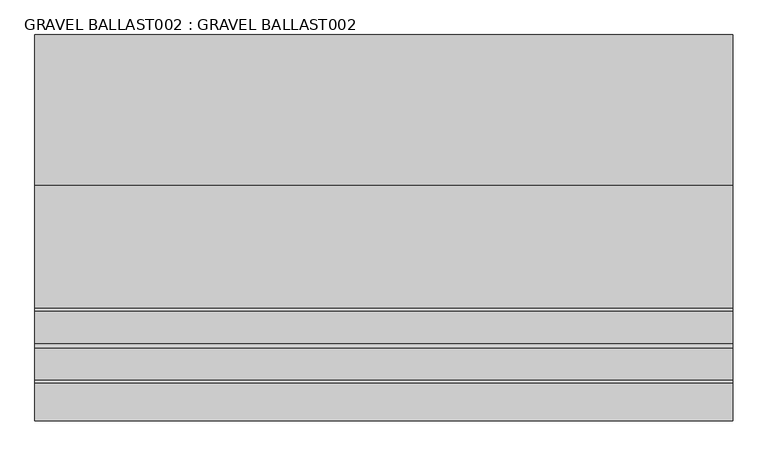
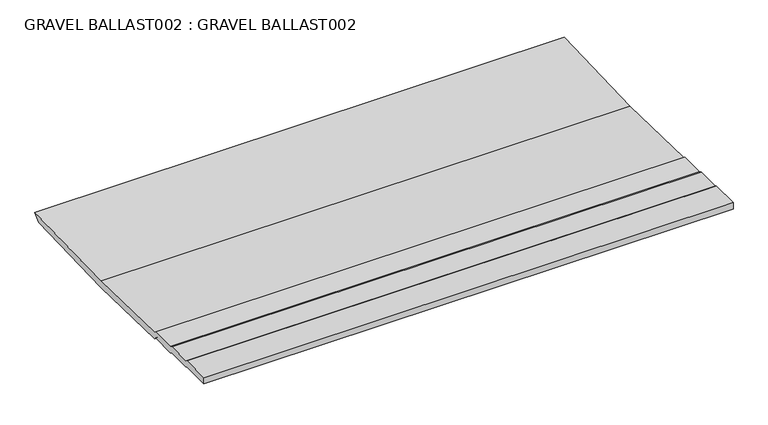
"""IFC4 building model written with IfcOpenShell, lengths in millimetres: proxy geometry, GRAVEL BALLAST002 : GRAVEL BALLAST002."""

import ifcopenshell
import ifcopenshell.guid

model = None  # the IFC model being written
_history = None  # IfcOwnerHistory: only IFC2X3 demands one
_inside = {}  # id of a spatial element -> (the spatial element, [elements in it])
_under = {}  # id of a project, library or spatial element -> (it, [spatial elements below it])
_declared = {}  # id of a project -> (the project, [libraries it declares])
_typed = {}  # id of a type object -> (the type object, [elements of that type])
_made_of = {}  # id of a material, layer set ... -> (it, [elements and type objects made of it])


def new_model(schema):
    """Start an empty IFC model of exactly this schema.

    Asked for "IFC4X3", IfcOpenShell would pick the latest addendum, in which some entities
    have other attributes; the version numbers below select the first issue.
    IFC2X3 requires an IfcOwnerHistory on every rooted entity: one is made here for all.
    """
    global model, _history
    if schema == "IFC4X3":
        model = ifcopenshell.file(schema_version=(4, 3, 0, 0))
    else:
        model = ifcopenshell.file(schema=schema)
    _inside.clear()
    _under.clear()
    _declared.clear()
    _typed.clear()
    _made_of.clear()
    _history = None
    if model.schema == "IFC2X3":
        org = make("IfcOrganization", Name="unknown")
        user = make(
            "IfcPersonAndOrganization",
            ThePerson=make("IfcPerson", FamilyName="unknown"),
            TheOrganization=org,
        )
        app = make(
            "IfcApplication",
            ApplicationDeveloper=org,
            Version="unknown",
            ApplicationFullName="unknown",
            ApplicationIdentifier="unknown",
        )
        _history = make(
            "IfcOwnerHistory",
            OwningUser=user,
            OwningApplication=app,
            ChangeAction="ADDED",
            CreationDate=0,
        )
    return model


def make(cls, **values):
    """One entity of the class cls with the attributes given. An attribute that is None is left unset."""
    return model.create_entity(
        cls, **{name: value for name, value in values.items() if value is not None}
    )


def rooted(cls, **values):
    """An entity with a GlobalId (a new one), such as an element, a storey or a relation."""
    return make(cls, GlobalId=ifcopenshell.guid.new(), OwnerHistory=_history, **values)


def si_unit(unit_type, name, prefix=None):
    """IfcSIUnit, for example si_unit("LENGTHUNIT", "METRE", prefix="MILLI")."""
    return make("IfcSIUnit", UnitType=unit_type, Prefix=prefix, Name=name)


def assignment(units):
    """IfcUnitAssignment: the units of a project."""
    return None if units is None else make("IfcUnitAssignment", Units=units)


def point(xyz):
    """IfcCartesianPoint."""
    return None if xyz is None else make("IfcCartesianPoint", Coordinates=xyz)


def direction(xyz):
    """IfcDirection."""
    return None if xyz is None else make("IfcDirection", DirectionRatios=xyz)


def frame(location, z_axis=None, x_axis=None):
    """IfcAxis2Placement3D, a coordinate frame: its origin and axes. An axis left out is left unset."""
    return make(
        "IfcAxis2Placement3D",
        Location=point(location),
        Axis=direction(z_axis),
        RefDirection=direction(x_axis),
    )


def origin():
    """The frame at (0, 0, 0) with its axes left unset."""
    return frame((0.0, 0.0, 0.0))


def place(relative_to, where):
    """IfcLocalPlacement: puts the frame where relative to a parent placement (None: the world)."""
    return make(
        "IfcLocalPlacement", PlacementRelTo=relative_to, RelativePlacement=where
    )


def context(
    kind, dimensions, precision=None, world=None, true_north=None, identifier=None
):
    """IfcGeometricRepresentationContext, for example the 3D "Model" context."""
    return make(
        "IfcGeometricRepresentationContext",
        ContextIdentifier=identifier,
        ContextType=kind,
        CoordinateSpaceDimension=dimensions,
        Precision=precision,
        WorldCoordinateSystem=world,
        TrueNorth=true_north,
    )


def project(units=None, contexts=None):
    """IfcProject with its units and contexts."""
    return rooted(
        "IfcProject",
        Name="project",
        RepresentationContexts=contexts,
        UnitsInContext=assignment(units),
    )


def spatial(cls, under=None, at=None, **own):
    """A site, building, storey or space (cls), placed at a placement, below another one or the project."""
    s = rooted(cls, ObjectPlacement=at, **own)
    if under is not None:
        _under.setdefault(under.id(), (under, []))[1].append(s)
    return s


def polyline(points):
    """IfcPolyline through the points."""
    return make("IfcPolyline", Points=[point(p) for p in points])


def outline(outer, holes=None, kind="AREA"):
    """IfcArbitraryClosedProfileDef: a profile drawn as a closed curve; with holes, ...WithVoids."""
    if holes is None:
        return make("IfcArbitraryClosedProfileDef", ProfileType=kind, OuterCurve=outer)
    return make(
        "IfcArbitraryProfileDefWithVoids",
        ProfileType=kind,
        OuterCurve=outer,
        InnerCurves=holes,
    )


def extrude(swept, where, along, depth):
    """IfcExtrudedAreaSolid: the profile swept, set in the frame where, extruded along a direction by depth."""
    return make(
        "IfcExtrudedAreaSolid",
        SweptArea=swept,
        Position=where,
        ExtrudedDirection=direction(along),
        Depth=depth,
    )


def shape(context_of_items, identifier, shape_type, items):
    """IfcShapeRepresentation: the items that make up one representation, for example the "Body"."""
    return make(
        "IfcShapeRepresentation",
        ContextOfItems=context_of_items,
        RepresentationIdentifier=identifier,
        RepresentationType=shape_type,
        Items=items,
    )


def source(mapping_origin, context_of_items, identifier, shape_type, items):
    """IfcRepresentationMap: a shape defined once, which mapped items show again and again."""
    return make(
        "IfcRepresentationMap",
        MappingOrigin=mapping_origin,
        MappedRepresentation=shape(context_of_items, identifier, shape_type, items),
    )


def transform(
    local_origin,
    x_axis=None,
    y_axis=None,
    z_axis=None,
    scale=None,
    scale2=None,
    scale3=None,
    uniform=True,
):
    """IfcCartesianTransformationOperator3D, or its non-uniform kind. x_axis, y_axis, z_axis: its Axis1, 2, 3."""
    if uniform:
        return make(
            "IfcCartesianTransformationOperator3D",
            Axis1=direction(x_axis),
            Axis2=direction(y_axis),
            LocalOrigin=point(local_origin),
            Scale=scale,
            Axis3=direction(z_axis),
        )
    return make(
        "IfcCartesianTransformationOperator3DnonUniform",
        Axis1=direction(x_axis),
        Axis2=direction(y_axis),
        LocalOrigin=point(local_origin),
        Scale=scale,
        Axis3=direction(z_axis),
        Scale2=scale2,
        Scale3=scale3,
    )


def mapped(mapping_source, mapping_target):
    """IfcMappedItem: shows the shape of a source again, moved by a transform."""
    return make(
        "IfcMappedItem", MappingSource=mapping_source, MappingTarget=mapping_target
    )


def made_of(thing, what):
    """Note that an element or type object is made of a material, layer set ...; save() writes the relation."""
    if what is not None:
        _made_of.setdefault(what.id(), (what, []))[1].append(thing)
    return thing


def element(
    cls,
    number,
    at=None,
    inside=None,
    cuts=None,
    type_object=None,
    material=None,
    context=None,
    identifier="Body",
    shape_type=None,
    held_by="IfcProductDefinitionShape",
    body=None,
    shapes=None,
    **own,
):
    """One element of the class cls, such as IfcWall. Its Tag is "e" and its number.

    at: its placement. inside: the storey or other place that contains it. cuts: it is an
    opening in that element (IfcRelVoidsElement). A single representation is given by context,
    identifier, shape_type and body (its items); several are given by shapes. held_by: the class
    of the entity that holds the representations. save() writes the other relations.
    """
    e = rooted(cls, Tag="e%d" % number, ObjectPlacement=at, **own)
    if body is not None:
        shapes = [shape(context, identifier, shape_type, body)]
    if shapes is not None:
        e.Representation = make(held_by, Representations=shapes)
    if inside is not None:
        _inside.setdefault(inside.id(), (inside, []))[1].append(e)
    if cuts is not None:
        rooted(
            "IfcRelVoidsElement", RelatingBuildingElement=cuts, RelatedOpeningElement=e
        )
    if type_object is not None:
        _typed.setdefault(type_object.id(), (type_object, []))[1].append(e)
    return made_of(e, material)


def aggregate(whole, parts):
    """IfcRelAggregates: a whole, such as a stair, and the parts it consists of."""
    return rooted("IfcRelAggregates", RelatingObject=whole, RelatedObjects=parts)


def save(model, path):
    """Write the relations noted so far, then the file.

    IfcRelAggregates (storeys below a building ...), IfcRelContainedInSpatialStructure (elements
    in a storey), IfcRelDefinesByType, IfcRelAssociatesMaterial and IfcRelDeclares: one each for
    every whole, place, type object, material and project.
    """
    for whole, parts in _under.values():
        aggregate(whole, parts)
    for where, things in _inside.values():
        rooted(
            "IfcRelContainedInSpatialStructure",
            RelatedElements=things,
            RelatingStructure=where,
        )
    for kind, things in _typed.values():
        rooted("IfcRelDefinesByType", RelatedObjects=things, RelatingType=kind)
    for what, things in _made_of.values():
        rooted("IfcRelAssociatesMaterial", RelatedObjects=things, RelatingMaterial=what)
    for by, libraries in _declared.values():
        rooted("IfcRelDeclares", RelatingContext=by, RelatedDefinitions=libraries)
    model.write(path)


def gravel_ballast002_gravel_ballast002_c19f6b3d(model_context):
    return source(origin(), model_context, "Body", "SweptSolid", [
        extrude(outline(polyline([(-5440.365918, 40253.79375), (-5549.8654297, 40253.79375), (-5549.8654297, 40278.5320313), (-5440.365918, 40278.5320313), (-5431.6554687, 40274.2507813), (-5341.0685547, 40274.2507813), (-5328.2239153, 40268.5233193), (-5234.272168, 40270.16875), (-5225.9987305, 40262.7585938), (-4873.4420898, 40254.5398438), (-4442.8393555, 40268.1982422), (-4468.0649414, 40242.9726562), (-4873.4420898, 40229.8015625), (-5225.9987305, 40238.0203125), (-5234.272168, 40245.4304687), (-5328.2239153, 40243.785038), (-5341.0685547, 40249.5125), (-5431.6554687, 40249.5125), (-5440.365918, 40253.79375)])), frame((12382.7678845, 0.0, 0.0), z_axis=(1.0, 0.0, 0.0), x_axis=(0.0, 1.0, 0.0)), (0.0, 0.0, 1.0), 2000.0),
    ])


if __name__ == "__main__":
    model = new_model("IFC4")
    model_context = context("Model", 3, world=origin())
    ifc_project = project(units=[si_unit("LENGTHUNIT", "METRE", prefix="MILLI")], contexts=[model_context])
    site = spatial("IfcSite", under=ifc_project)
    building = spatial("IfcBuilding", under=site)
    placement = place(None, origin())
    gravel_ballast002_gravel_ballast002_shape = gravel_ballast002_gravel_ballast002_c19f6b3d(model_context)
    element("IfcBuildingElementProxy", 1, Name="GRAVEL BALLAST002 : GRAVEL BALLAST002", ObjectType="GRAVEL BALLAST002 : GRAVEL BALLAST002", at=placement, inside=building, context=model_context, shape_type="MappedRepresentation", body=[
        mapped(gravel_ballast002_gravel_ballast002_shape, transform((0.0, 0.0, 0.0), x_axis=(1.0, 0.0, 0.0), y_axis=(0.0, 1.0, 0.0), z_axis=(0.0, 0.0, 1.0))),
    ])
    save(model, "model.ifc")

# Revit data of these elements
# Type "GRAVEL BALLAST002 : GRAVEL BALLAST002"
#   NameOverride = "GRAVEL BALLAST002"
# Element 1 (IfcBuildingElementProxy, "GRAVEL BALLAST002 : GRAVEL BALLAST002")
#   Materials on its faces: "GRAVEL BALLAST"
# Materials
#   "GRAVEL BALLAST": class "Unassigned", colour RGB 128 128 128, transparency 0, Cost = 0
